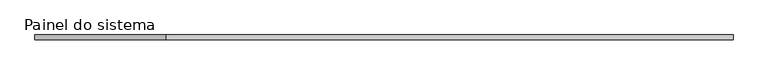
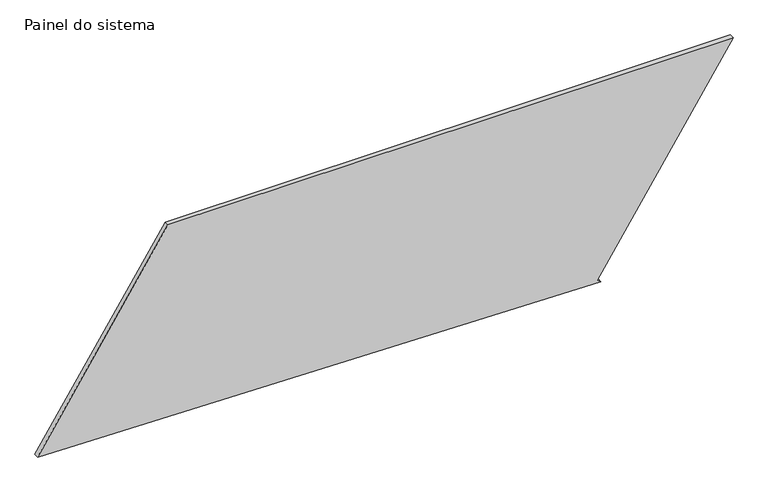
"""IFC4 building model written with IfcOpenShell, lengths in millimetres: plate geometry, Painel do sistema : Envidraçado."""

from ifc_helpers import new_model, si_unit, frame, origin, place, context, project, spatial, polyline, outline, extrude, source, transform, mapped, element, save


def painel_do_sistema_16acd4ef(model_context):
    return source(origin(), model_context, "Body", "SweptSolid", [
        extrude(outline(polyline([(0.0, 1159.0863303), (13.6354654, 1138.1322356), (1137.9109441, 1869.732414), (1137.9109441, -1169.8035262), (62.3058409, -1869.732414), (0.0, 1159.0863303)])), frame((0.0, 24.5, 0.0), z_axis=(0.0, 1.0, 0.0), x_axis=(0.0, 0.0, 1.0)), (0.0, 0.0, 1.0), 25.0),
    ])


if __name__ == "__main__":
    model = new_model("IFC4")
    model_context = context("Model", 3, world=origin())
    ifc_project = project(units=[si_unit("LENGTHUNIT", "METRE", prefix="MILLI")], contexts=[model_context])
    site = spatial("IfcSite", under=ifc_project)
    building = spatial("IfcBuilding", under=site)
    placement = place(None, origin())
    painel_do_sistema_shape = painel_do_sistema_16acd4ef(model_context)
    element("IfcPlate", 1, ObjectType="Painel do sistema : Envidraçado", at=placement, inside=building, context=model_context, shape_type="MappedRepresentation", body=[
        mapped(painel_do_sistema_shape, transform((0.0, 0.0, 0.0), x_axis=(1.0, 0.0, 0.0), y_axis=(0.0, 1.0, 0.0), z_axis=(0.0, 0.0, 1.0))),
    ])
    save(model, "model.ifc")

# Revit data of these elements
# Type "Painel do sistema : Envidraçado"
#   Construction Type Id = "GSP4R"
#   Analytic Construction = "Vidraça única Pilkington 1/8 pol"
#   Visual Light Transmittance = 0.9
#   Solar Heat Gain Coefficient = 0.86
#   Heat Transfer Coefficient (U) = 6.7069 W/(m²·K)
# Element 1 (IfcPlate, "Painel do sistema : Envidraçado")
#   Materials on its faces: "Vidro"
# Materials
#   "Vidro": class "Vidro", colour RGB 0 128 192, transparency 0.9, Description = "Vidro de sílica", Cost = 0
